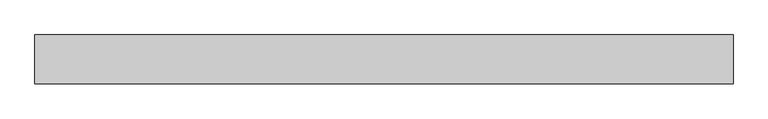
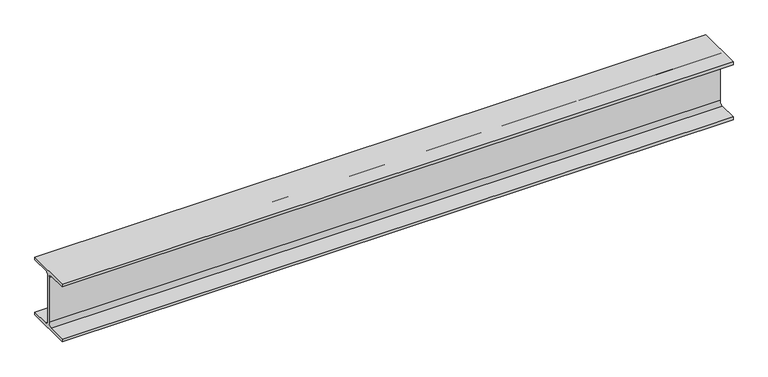
"""IFC4 building model written with IfcOpenShell, lengths in millimetres: beam geometry, 0912_Steel Framing_H-KSD3502 : H_SB_ASB_H-194x150x6x9."""

from ifc_helpers import new_model, si_unit, point, frame, frame_2d, origin, place, context, project, spatial, polyline, circle_curve, trimmed, segment, composite_curve, outline, extrude, source, transform, mapped, element, save


def beam_15ee70ce(model_context):
    return source(origin(), model_context, "Body", "SweptSolid", [
        extrude(outline(composite_curve([segment(polyline([(-75.0, -88.0), (-16.0, -88.0)]), True, "CONTINUOUS"), segment(trimmed(circle_curve(frame_2d((-16.0, -75.0)), 13.0), [point((-16.0, -88.0))], [point((-3.0, -75.0))], True, "CARTESIAN"), True, "CONTINUOUS"), segment(polyline([(-3.0, -75.0), (-3.0, 75.0)]), True, "CONTINUOUS"), segment(trimmed(circle_curve(frame_2d((-16.0, 75.0)), 13.0), [point((-3.0, 75.0))], [point((-16.0, 88.0))], True, "CARTESIAN"), True, "CONTINUOUS"), segment(polyline([(-16.0, 88.0), (-75.0, 88.0), (-75.0, 97.0), (75.0, 97.0), (75.0, 88.0), (16.0, 88.0)]), True, "CONTINUOUS"), segment(trimmed(circle_curve(frame_2d((16.0, 75.0)), 13.0), [point((16.0, 88.0))], [point((3.0, 75.0))], True, "CARTESIAN"), True, "CONTINUOUS"), segment(polyline([(3.0, 75.0), (3.0, -75.0)]), True, "CONTINUOUS"), segment(trimmed(circle_curve(frame_2d((16.0, -75.0)), 13.0), [point((3.0, -75.0))], [point((16.0, -88.0))], True, "CARTESIAN"), True, "CONTINUOUS"), segment(polyline([(16.0, -88.0), (75.0, -88.0), (75.0, -97.0), (-75.0, -97.0), (-75.0, -88.0)]), True, "CONTINUOUS")], self_intersect=False)), frame((-1067.7446443, 0.0, 0.0), z_axis=(1.0, 0.0, 0.0), x_axis=(0.0, 1.0, 0.0)), (0.0, 0.0, 1.0), 2135.4892885),
    ])


if __name__ == "__main__":
    model = new_model("IFC4")
    model_context = context("Model", 3, world=origin())
    ifc_project = project(units=[si_unit("LENGTHUNIT", "METRE", prefix="MILLI")], contexts=[model_context])
    site = spatial("IfcSite", under=ifc_project)
    building = spatial("IfcBuilding", under=site)
    placement = place(None, origin())
    beam_shape = beam_15ee70ce(model_context)
    element("IfcBeam", 1, ObjectType="0912_Steel Framing_H-KSD3502 : H_SB_ASB_H-194x150x6x9", at=placement, inside=building, context=model_context, shape_type="MappedRepresentation", body=[
        mapped(beam_shape, transform((0.0, 0.0, 0.0), x_axis=(1.0, 0.0, 0.0), y_axis=(0.0, 1.0, 0.0), z_axis=(0.0, 0.0, 1.0))),
    ])
    save(model, "model.ifc")

# Revit data of these elements
# Type "0912_Steel Framing_H-KSD3502 : H_SB_ASB_H-194x150x6x9"
#   H_WM Code_1 = "S01AA002-00001 | Main Steel Structure Fabrication Work | Shelter/Building | Medium Steel - Standard (90KG/M>Weight≥30KG/M) | Material: (   )"
#   H_WM Code_2 = "S03AA028-00001 | Main Steel Structure Erection Work | Shelter/Building | Medium Steel (90KG/M>Weight≥30KG/M) | Material: (   )"
#   H_WM Code_3 = "S01AA010-00001 | Main Steel Structure Fabrication Work | Shelter/Building | Steel Painting/Coating | for Non-Fireproofed Steel Surface, Surface Preparation, Primer, Second & Final Coat | Material: (   )"
#   H_Q'ty Cal Type Tag = "SB-Q2"
#   Width = 15.0 cm
#   Web Thickness = 0.6 cm
#   Web Fillet = 1.3 cm
#   Warping Constant = 43316.0 cm⁶
#   W = 0
#   Torsional Moment of Inertia = 8.622 cm⁴
#   Section Area = 39.01 cm²
#   Plastic Modulus weak axis = 104.0 cm³
#   Plastic Modulus strong axis = 309.0 cm³
#   Perimeter = 0.95 m²/m
#   Nominal Weight = 30.60 kgf/m
#   Moment of Inertia weak axis = 507.00 cm⁴
#   Moment of Inertia strong axis = 2690.00 cm⁴
#   Height = 19.4 cm
#   Flange Thickness = 0.9 cm
#   Elastic Modulus weak axis = 67.6 cm³
#   Elastic Modulus strong axis = 277.0 cm³
#   Centroid Vertical = 9.7 cm
#   Centroid Horizontal = 7.5 cm
#   Ix = 26900000
#   Length [instance default] = 1.5240 m
#   Zx = 309000
#   b = 0.1500 m
#   h = 0.1940 m
#   r = 0.0130 m
#   s = 0.0060 m
#   t = 0.0090 m
#   A = 0.003901 m²
#   Structural Material [instance default] = Steel, 45-345
#   Assembly Code = ""
# Element 1 (IfcBeam, "0912_Steel Framing_H-KSD3502 : H_SB_ASB_H-194x150x6x9")
#   Structural Material = none
# Materials
#   "Steel, 45-345": class "Metal", colour RGB 189 187 185, transparency 0, Description = "Steel 345 MPa", Cost = 0
